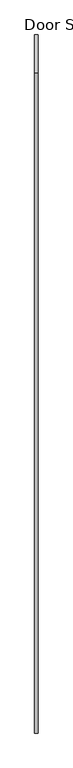
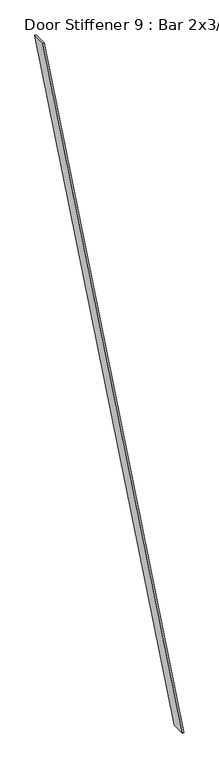
"""IFC4 building model written with IfcOpenShell, lengths in millimetres: proxy geometry, Door Stiffener 9 : Bar 2x3/16."""

from ifc_helpers import new_model, si_unit, frame, origin, place, context, project, spatial, polyline, outline, extrude, source, transform, mapped, element, save


def door_stiffener_9_bar_2x3_16_34f525c1(model_context):
    return source(origin(), model_context, "Body", "SweptSolid", [
        extrude(outline(polyline([(-534200.9077829, 2400.3), (-534145.8788841, 2400.3), (-535108.4374853, 88.9), (-535163.4663841, 88.9), (-534200.9077829, 2400.3)])), frame((587403.9934739, 0.0, 0.0), z_axis=(1.0, 0.0, 0.0), x_axis=(0.0, 1.0, 0.0)), (0.0, 0.0, 1.0), 4.7625),
    ])


if __name__ == "__main__":
    model = new_model("IFC4")
    model_context = context("Model", 3, world=origin())
    ifc_project = project(units=[si_unit("LENGTHUNIT", "METRE", prefix="MILLI")], contexts=[model_context])
    site = spatial("IfcSite", under=ifc_project)
    building = spatial("IfcBuilding", under=site)
    placement = place(None, origin())
    door_stiffener_9_bar_2x3_16_shape = door_stiffener_9_bar_2x3_16_34f525c1(model_context)
    element("IfcBuildingElementProxy", 1, Name="Door Stiffener 9 : Bar 2x3/16", ObjectType="Door Stiffener 9 : Bar 2x3/16", at=placement, inside=building, context=model_context, shape_type="MappedRepresentation", body=[
        mapped(door_stiffener_9_bar_2x3_16_shape, transform((0.0, 0.0, 0.0), x_axis=(1.0, 0.0, 0.0), y_axis=(0.0, 1.0, 0.0), z_axis=(0.0, 0.0, 1.0))),
    ])
    save(model, "model.ifc")

# Revit data of these elements
# Element 1 (IfcBuildingElementProxy, "Door Stiffener 9 : Bar 2x3/16")
#   Materials on its faces: "2\"X3/16\" GALV. STL BAR STOCK"
# Materials
#   "2\"X3/16\" GALV. STL BAR STOCK": class "Generic", colour RGB 211 211 207, transparency 0, Cost = 0
